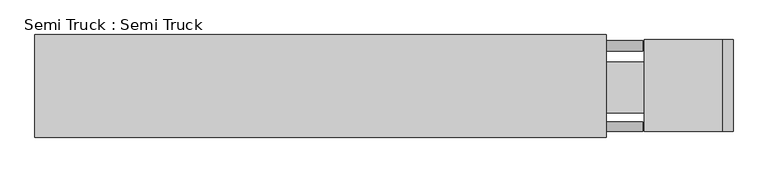
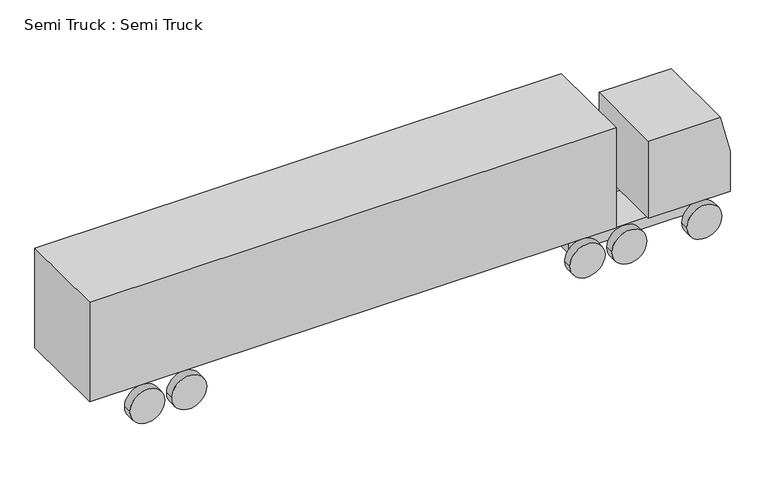
"""IFC4 building model written with IfcOpenShell, lengths in millimetres: proxy geometry, Semi Truck : Semi Truck."""

from ifc_helpers import new_model, si_unit, point, frame, frame_2d, origin, place, context, project, spatial, polyline, circle_curve, trimmed, segment, composite_curve, outline, extrude, source, transform, mapped, element, save


def semi_truck_semi_truck_f452f70d(model_context):
    return source(origin(), model_context, "Body", "SweptSolid", [
        extrude(outline(polyline([(12801.9874353, 1803.4), (16129.3874353, 1803.4), (16129.3874353, 584.2), (12801.9874353, 584.2), (12801.9874353, 1803.4)])), frame((0.0, 0.0, 474.4382453), z_axis=(0.0, 0.0, 1.0), x_axis=(1.0, 0.0, 0.0)), (0.0, 0.0, 1.0), 279.4),
        extrude(outline(composite_curve([segment(trimmed(circle_curve(frame_2d((462.8573069, 16091.7081812)), 457.2), [point((462.8573069, 16548.9081812))], [point((462.8573069, 15634.5081812))], False, "CARTESIAN"), True, "CONTINUOUS"), segment(trimmed(circle_curve(frame_2d((462.8573069, 16091.7081812)), 457.2), [point((462.8573069, 15634.5081812))], [point((462.8573069, 16548.9081812))], False, "CARTESIAN"), True, "CONTINUOUS")], self_intersect=False)), frame((0.0, 133.878403, 0.0), z_axis=(0.0, 1.0, 0.0), x_axis=(0.0, 0.0, 1.0)), (0.0, 0.0, 1.0), 228.6),
        extrude(outline(composite_curve([segment(trimmed(circle_curve(frame_2d((464.8502402, 13047.865337)), 457.2), [point((464.8502402, 13505.065337))], [point((464.8502402, 12590.665337))], False, "CARTESIAN"), True, "CONTINUOUS"), segment(trimmed(circle_curve(frame_2d((464.8502402, 13047.865337)), 457.2), [point((464.8502402, 12590.665337))], [point((464.8502402, 13505.065337))], False, "CARTESIAN"), True, "CONTINUOUS")], self_intersect=False)), frame((0.0, 133.878403, 0.0), z_axis=(0.0, 1.0, 0.0), x_axis=(0.0, 0.0, 1.0)), (0.0, 0.0, 1.0), 228.6),
        extrude(outline(composite_curve([segment(trimmed(circle_curve(frame_2d((462.8573069, 14137.8642567)), 457.2), [point((462.8573069, 14595.0642567))], [point((462.8573069, 13680.6642567))], False, "CARTESIAN"), True, "CONTINUOUS"), segment(trimmed(circle_curve(frame_2d((462.8573069, 14137.8642567)), 457.2), [point((462.8573069, 13680.6642567))], [point((462.8573069, 14595.0642567))], False, "CARTESIAN"), True, "CONTINUOUS")], self_intersect=False)), frame((0.0, 133.878403, 0.0), z_axis=(0.0, 1.0, 0.0), x_axis=(0.0, 0.0, 1.0)), (0.0, 0.0, 1.0), 228.6),
        extrude(outline(composite_curve([segment(trimmed(circle_curve(frame_2d((471.1409074, 2673.3437978)), 457.2), [point((471.1409074, 3130.5437978))], [point((471.1409074, 2216.1437978))], False, "CARTESIAN"), True, "CONTINUOUS"), segment(trimmed(circle_curve(frame_2d((471.1409074, 2673.3437978)), 457.2), [point((471.1409074, 2216.1437978))], [point((471.1409074, 3130.5437978))], False, "CARTESIAN"), True, "CONTINUOUS")], self_intersect=False)), frame((0.0, 133.878403, 0.0), z_axis=(0.0, 1.0, 0.0), x_axis=(0.0, 0.0, 1.0)), (0.0, 0.0, 1.0), 228.6),
        extrude(outline(polyline([(1066.8, 16764.0), (2168.2557891, 16764.0), (3200.4, 16501.4938374), (3200.4, 14630.4), (1066.8, 14630.4), (1066.8, 16764.0)])), frame((0.0, 133.878403, 0.0), z_axis=(0.0, 1.0, 0.0), x_axis=(0.0, 0.0, 1.0)), (0.0, 0.0, 1.0), 2212.0834331),
        extrude(outline(composite_curve([segment(trimmed(circle_curve(frame_2d((461.9942506, 16091.7889873)), 457.2), [point((461.9942506, 16548.9889873))], [point((461.9942506, 15634.5889873))], False, "CARTESIAN"), True, "CONTINUOUS"), segment(trimmed(circle_curve(frame_2d((461.9942506, 16091.7889873)), 457.2), [point((461.9942506, 15634.5889873))], [point((461.9942506, 16548.9889873))], False, "CARTESIAN"), True, "CONTINUOUS")], self_intersect=False)), frame((0.0, 2066.561836, 0.0), z_axis=(0.0, 1.0, 0.0), x_axis=(0.0, 0.0, 1.0)), (0.0, 0.0, 1.0), 254.0),
        extrude(outline(composite_curve([segment(trimmed(circle_curve(frame_2d((471.1409074, 2673.3437978)), 457.2), [point((471.1409074, 3130.5437978))], [point((471.1409074, 2216.1437978))], False, "CARTESIAN"), True, "CONTINUOUS"), segment(trimmed(circle_curve(frame_2d((471.1409074, 2673.3437978)), 457.2), [point((471.1409074, 2216.1437978))], [point((471.1409074, 3130.5437978))], False, "CARTESIAN"), True, "CONTINUOUS")], self_intersect=False)), frame((0.0, 133.878403, 0.0), z_axis=(0.0, 1.0, 0.0), x_axis=(0.0, 0.0, 1.0)), (0.0, 0.0, 1.0), 228.6),
        extrude(outline(composite_curve([segment(trimmed(circle_curve(frame_2d((471.1409074, 1581.3519448)), 457.2), [point((471.1409074, 2038.5519448))], [point((471.1409074, 1124.1519448))], False, "CARTESIAN"), True, "CONTINUOUS"), segment(trimmed(circle_curve(frame_2d((471.1409074, 1581.3519448)), 457.2), [point((471.1409074, 1124.1519448))], [point((471.1409074, 2038.5519448))], False, "CARTESIAN"), True, "CONTINUOUS")], self_intersect=False)), frame((0.0, 133.878403, 0.0), z_axis=(0.0, 1.0, 0.0), x_axis=(0.0, 0.0, 1.0)), (0.0, 0.0, 1.0), 228.6),
        extrude(outline(composite_curve([segment(trimmed(circle_curve(frame_2d((464.0721679, 13049.2660873)), 457.2), [point((464.0721679, 13506.4660873))], [point((464.0721679, 12592.0660873))], False, "CARTESIAN"), True, "CONTINUOUS"), segment(trimmed(circle_curve(frame_2d((464.0721679, 13049.2660873)), 457.2), [point((464.0721679, 12592.0660873))], [point((464.0721679, 13506.4660873))], False, "CARTESIAN"), True, "CONTINUOUS")], self_intersect=False)), frame((0.0, 2066.561836, 0.0), z_axis=(0.0, 1.0, 0.0), x_axis=(0.0, 0.0, 1.0)), (0.0, 0.0, 1.0), 254.0),
        extrude(outline(composite_curve([segment(trimmed(circle_curve(frame_2d((464.0721679, 14141.2579404)), 457.2), [point((464.0721679, 14598.4579404))], [point((464.0721679, 13684.0579404))], False, "CARTESIAN"), True, "CONTINUOUS"), segment(trimmed(circle_curve(frame_2d((464.0721679, 14141.2579404)), 457.2), [point((464.0721679, 13684.0579404))], [point((464.0721679, 14598.4579404))], False, "CARTESIAN"), True, "CONTINUOUS")], self_intersect=False)), frame((0.0, 2066.561836, 0.0), z_axis=(0.0, 1.0, 0.0), x_axis=(0.0, 0.0, 1.0)), (0.0, 0.0, 1.0), 254.0),
        extrude(outline(composite_curve([segment(trimmed(circle_curve(frame_2d((471.1409074, 1581.3519448)), 457.2), [point((471.1409074, 2038.5519448))], [point((471.1409074, 1124.1519448))], False, "CARTESIAN"), True, "CONTINUOUS"), segment(trimmed(circle_curve(frame_2d((471.1409074, 1581.3519448)), 457.2), [point((471.1409074, 1124.1519448))], [point((471.1409074, 2038.5519448))], False, "CARTESIAN"), True, "CONTINUOUS")], self_intersect=False)), frame((0.0, 2066.561836, 0.0), z_axis=(0.0, 1.0, 0.0), x_axis=(0.0, 0.0, 1.0)), (0.0, 0.0, 1.0), 254.0),
        extrude(outline(composite_curve([segment(trimmed(circle_curve(frame_2d((471.1409074, 2673.3437978)), 457.2), [point((471.1409074, 3130.5437978))], [point((471.1409074, 2216.1437978))], False, "CARTESIAN"), True, "CONTINUOUS"), segment(trimmed(circle_curve(frame_2d((471.1409074, 2673.3437978)), 457.2), [point((471.1409074, 2216.1437978))], [point((471.1409074, 3130.5437978))], False, "CARTESIAN"), True, "CONTINUOUS")], self_intersect=False)), frame((0.0, 2066.561836, 0.0), z_axis=(0.0, 1.0, 0.0), x_axis=(0.0, 0.0, 1.0)), (0.0, 0.0, 1.0), 254.0),
        extrude(outline(polyline([(13716.0, 2463.8), (13716.0, 0.0), (0.0, 0.0), (0.0, 2463.8), (13716.0, 2463.8)])), frame((0.0, 0.0, 1219.2), z_axis=(0.0, 0.0, 1.0), x_axis=(1.0, 0.0, 0.0)), (0.0, 0.0, 1.0), 2743.2),
    ])


if __name__ == "__main__":
    model = new_model("IFC4")
    model_context = context("Model", 3, world=origin())
    ifc_project = project(units=[si_unit("LENGTHUNIT", "METRE", prefix="MILLI")], contexts=[model_context])
    site = spatial("IfcSite", under=ifc_project)
    building = spatial("IfcBuilding", under=site)
    placement = place(None, origin())
    semi_truck_semi_truck_shape = semi_truck_semi_truck_f452f70d(model_context)
    element("IfcBuildingElementProxy", 1, Name="Semi Truck : Semi Truck", ObjectType="Semi Truck : Semi Truck", at=placement, inside=building, context=model_context, shape_type="MappedRepresentation", body=[
        mapped(semi_truck_semi_truck_shape, transform((0.0, 0.0, 0.0), x_axis=(1.0, 0.0, 0.0), y_axis=(0.0, 1.0, 0.0), z_axis=(0.0, 0.0, 1.0))),
    ])
    save(model, "model.ifc")

# Revit data of these elements
# Type "Semi Truck : Semi Truck"
#   Height = 0
